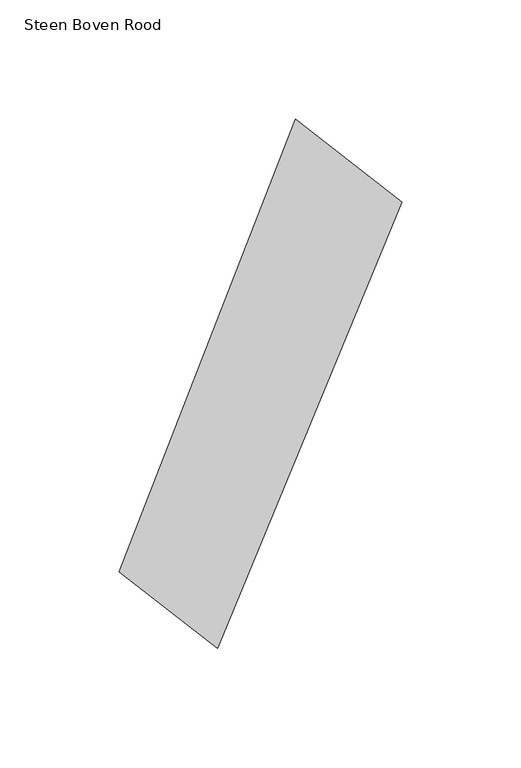
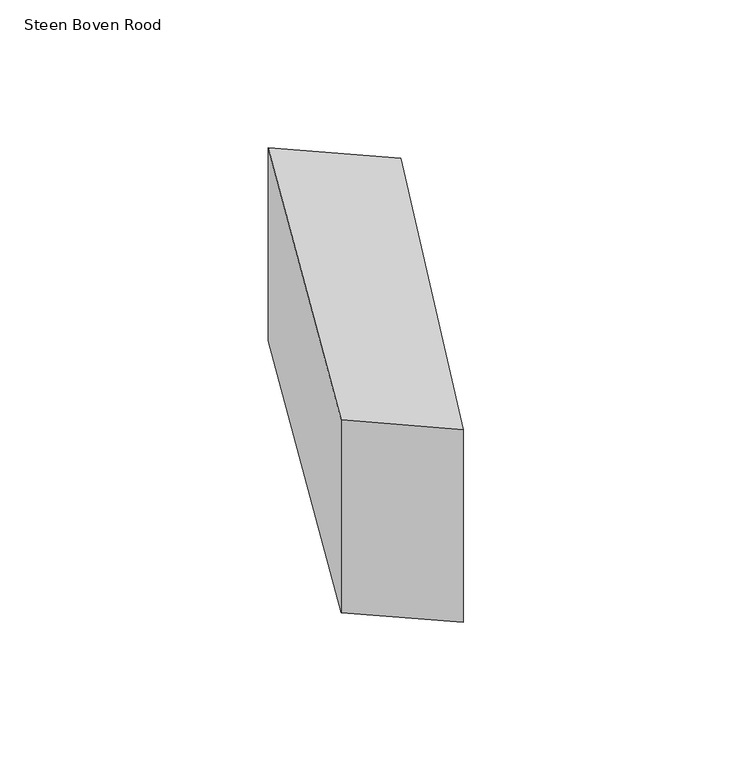
"""IFC4 building model written with IfcOpenShell, lengths in millimetres: proxy geometry, 00_GMA_steen_versie_4 : Steen Boven Rood."""

from ifc_helpers import new_model, si_unit, origin, origin_with_axes, place, context, project, spatial, polyline, outline, extrude, source, transform, mapped, element, save


def steen_boven_rood_319390fa(model_context):
    return source(origin(), model_context, "Body", "SweptSolid", [
        extrude(outline(polyline([(141.247189, 167.5928483), (63.8843685, -19.627819), (22.6264199, 12.5473646), (96.5781494, 202.4610001), (141.247189, 167.5928483)])), origin_with_axes(), (0.0, 0.0, 1.0), 100.0),
    ])


if __name__ == "__main__":
    model = new_model("IFC4")
    model_context = context("Model", 3, world=origin())
    ifc_project = project(units=[si_unit("LENGTHUNIT", "METRE", prefix="MILLI")], contexts=[model_context])
    site = spatial("IfcSite", under=ifc_project)
    building = spatial("IfcBuilding", under=site)
    placement = place(None, origin())
    steen_boven_rood_shape = steen_boven_rood_319390fa(model_context)
    element("IfcBuildingElementProxy", 1, Name="00_GMA_steen_versie_4 : Steen Boven Rood", ObjectType="00_GMA_steen_versie_4 : Steen Boven Rood", at=placement, inside=building, context=model_context, shape_type="MappedRepresentation", body=[
        mapped(steen_boven_rood_shape, transform((0.0, 0.0, 0.0), x_axis=(1.0, 0.0, 0.0), y_axis=(0.0, 1.0, 0.0), z_axis=(0.0, 0.0, 1.0))),
    ])
    save(model, "model.ifc")

# Revit data of these elements
# Type "00_GMA_steen_versie_4 : Steen Boven Rood"
#   StootVoegHalfBoven [instance default] = 5 mm
#   StootVoegHalf [instance default] = 5 mm
#   StootVoegBreedteOnder = 10 mm
#   StootVoegBreedteBoven = 10 mm
#   Steendikte = 100 mm
#   LintVoegOnderHalf = 5 mm
#   LintVoegOnder = 10 mm
#   LintVoegBovenHalf = 0 mm
#   LintVoegBoven = 0 mm
#   materiaal = 21_steen_rood
#   MateriaalVoeg = none
#   Default Elevation = 0
# Element 1 (IfcBuildingElementProxy, "00_GMA_steen_versie_4 : Steen Boven Rood")
#   Materials on its faces: "21_steen_rood"
# Materials
#   "21_steen_rood": class "Unassigned", colour RGB 213 111 43, transparency 0, Cost = 0
